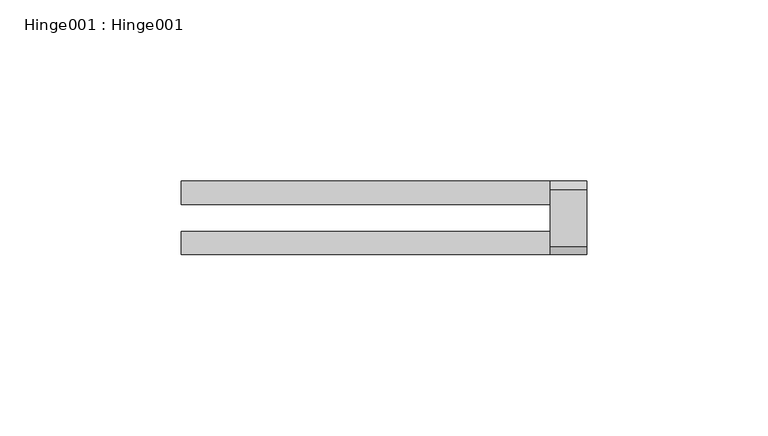
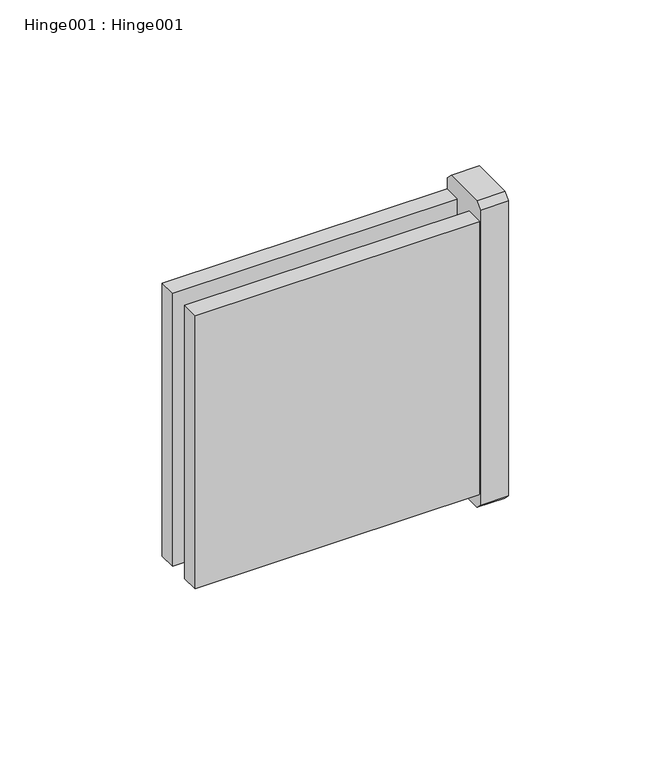
"""IFC4 building model written with IfcOpenShell, lengths in millimetres: proxy geometry, Hinge001 : Hinge001."""

from ifc_helpers import new_model, si_unit, frame, origin, place, context, project, spatial, polyline, outline, extrude, source, transform, mapped, element, save


def hinge001_hinge001_0a1b6b46(model_context):
    return source(origin(), model_context, "Body", "SweptSolid", [
        extrude(outline(polyline([(9646.679882, 37769.0012561), (9630.9579547, 37769.0012561), (9628.7124545, 37771.2467563), (9628.7124545, 37882.1452438), (9630.9579547, 37884.3907439), (9646.679882, 37884.3907439), (9648.924946, 37882.1456799), (9648.924946, 37771.2463201), (9646.679882, 37769.0012561)])), frame((-9232.0719278, 0.0, 0.0), z_axis=(1.0, 0.0, 0.0), x_axis=(0.0, 1.0, 0.0)), (0.0, 0.0, 1.0), 10.0),
        extrude(outline(polyline([(-9333.6719278, 9642.574946), (-9333.6719278, 9648.924946), (-9232.0719278, 9648.924946), (-9232.0719278, 9642.574946), (-9333.6719278, 9642.574946)])), frame((0.0, 0.0, 37775.3512561), z_axis=(0.0, 0.0, 1.0), x_axis=(1.0, 0.0, 0.0)), (0.0, 0.0, 1.0), 102.6894878),
        extrude(outline(polyline([(-9333.6719278, 9628.7124545), (-9333.6719278, 9635.0624545), (-9232.0719278, 9635.0624545), (-9232.0719278, 9628.7124545), (-9333.6719278, 9628.7124545)])), frame((0.0, 0.0, 37775.3512561), z_axis=(0.0, 0.0, 1.0), x_axis=(1.0, 0.0, 0.0)), (0.0, 0.0, 1.0), 102.6894878),
    ])


if __name__ == "__main__":
    model = new_model("IFC4")
    model_context = context("Model", 3, world=origin())
    ifc_project = project(units=[si_unit("LENGTHUNIT", "METRE", prefix="MILLI")], contexts=[model_context])
    site = spatial("IfcSite", under=ifc_project)
    building = spatial("IfcBuilding", under=site)
    placement = place(None, origin())
    hinge001_hinge001_shape = hinge001_hinge001_0a1b6b46(model_context)
    element("IfcBuildingElementProxy", 1, Name="Hinge001 : Hinge001", ObjectType="Hinge001 : Hinge001", at=placement, inside=building, context=model_context, shape_type="MappedRepresentation", body=[
        mapped(hinge001_hinge001_shape, transform((0.0, 0.0, 0.0), x_axis=(1.0, 0.0, 0.0), y_axis=(0.0, 1.0, 0.0), z_axis=(0.0, 0.0, 1.0))),
    ])
    save(model, "model.ifc")

# Revit data of these elements
# Type "Hinge001 : Hinge001"
#   NameOverride = "Hinge001"
# Element 1 (IfcBuildingElementProxy, "Hinge001 : Hinge001")
#   Materials on its faces: "HEAVY DUTY STAINLESS STEEL HINGE (90 DEGREE ROTATION)"
# Materials
#   "HEAVY DUTY STAINLESS STEEL HINGE (90 DEGREE ROTATION)": class "Unassigned", colour RGB 128 128 128, transparency 0
